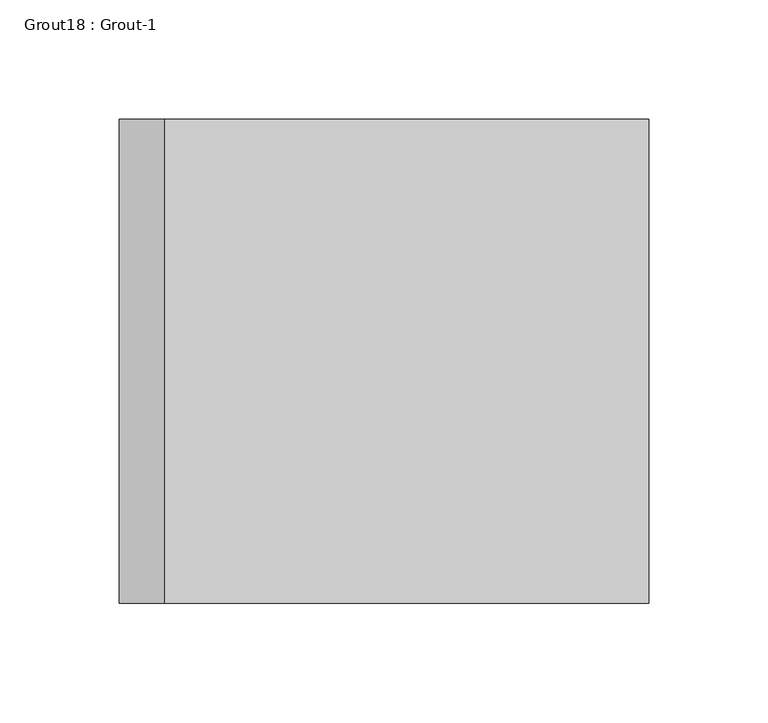
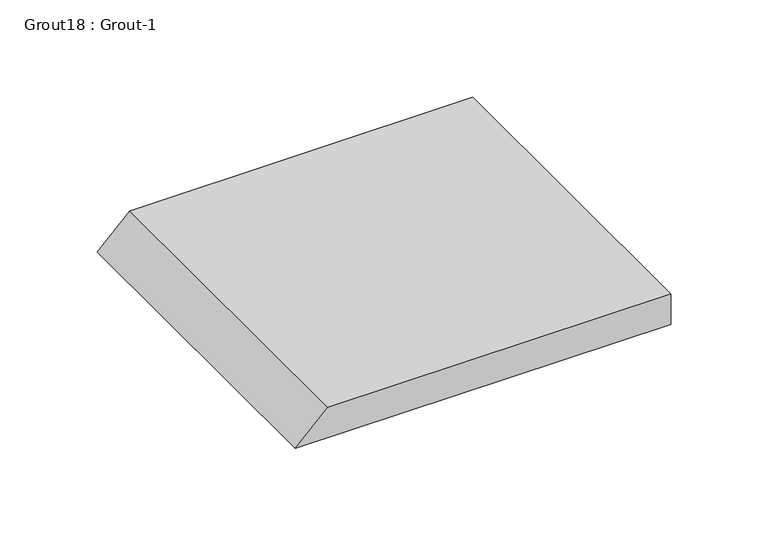
"""IFC4 building model written with IfcOpenShell, lengths in millimetres: proxy geometry, Grout18 : Grout-1."""

import ifcopenshell
import ifcopenshell.guid

model = None  # the IFC model being written
_history = None  # IfcOwnerHistory: only IFC2X3 demands one
_inside = {}  # id of a spatial element -> (the spatial element, [elements in it])
_under = {}  # id of a project, library or spatial element -> (it, [spatial elements below it])
_declared = {}  # id of a project -> (the project, [libraries it declares])
_typed = {}  # id of a type object -> (the type object, [elements of that type])
_made_of = {}  # id of a material, layer set ... -> (it, [elements and type objects made of it])


def new_model(schema):
    """Start an empty IFC model of exactly this schema.

    Asked for "IFC4X3", IfcOpenShell would pick the latest addendum, in which some entities
    have other attributes; the version numbers below select the first issue.
    IFC2X3 requires an IfcOwnerHistory on every rooted entity: one is made here for all.
    """
    global model, _history
    if schema == "IFC4X3":
        model = ifcopenshell.file(schema_version=(4, 3, 0, 0))
    else:
        model = ifcopenshell.file(schema=schema)
    _inside.clear()
    _under.clear()
    _declared.clear()
    _typed.clear()
    _made_of.clear()
    _history = None
    if model.schema == "IFC2X3":
        org = make("IfcOrganization", Name="unknown")
        user = make(
            "IfcPersonAndOrganization",
            ThePerson=make("IfcPerson", FamilyName="unknown"),
            TheOrganization=org,
        )
        app = make(
            "IfcApplication",
            ApplicationDeveloper=org,
            Version="unknown",
            ApplicationFullName="unknown",
            ApplicationIdentifier="unknown",
        )
        _history = make(
            "IfcOwnerHistory",
            OwningUser=user,
            OwningApplication=app,
            ChangeAction="ADDED",
            CreationDate=0,
        )
    return model


def make(cls, **values):
    """One entity of the class cls with the attributes given. An attribute that is None is left unset."""
    return model.create_entity(
        cls, **{name: value for name, value in values.items() if value is not None}
    )


def rooted(cls, **values):
    """An entity with a GlobalId (a new one), such as an element, a storey or a relation."""
    return make(cls, GlobalId=ifcopenshell.guid.new(), OwnerHistory=_history, **values)


def si_unit(unit_type, name, prefix=None):
    """IfcSIUnit, for example si_unit("LENGTHUNIT", "METRE", prefix="MILLI")."""
    return make("IfcSIUnit", UnitType=unit_type, Prefix=prefix, Name=name)


def assignment(units):
    """IfcUnitAssignment: the units of a project."""
    return None if units is None else make("IfcUnitAssignment", Units=units)


def point(xyz):
    """IfcCartesianPoint."""
    return None if xyz is None else make("IfcCartesianPoint", Coordinates=xyz)


def direction(xyz):
    """IfcDirection."""
    return None if xyz is None else make("IfcDirection", DirectionRatios=xyz)


def frame(location, z_axis=None, x_axis=None):
    """IfcAxis2Placement3D, a coordinate frame: its origin and axes. An axis left out is left unset."""
    return make(
        "IfcAxis2Placement3D",
        Location=point(location),
        Axis=direction(z_axis),
        RefDirection=direction(x_axis),
    )


def origin():
    """The frame at (0, 0, 0) with its axes left unset."""
    return frame((0.0, 0.0, 0.0))


def place(relative_to, where):
    """IfcLocalPlacement: puts the frame where relative to a parent placement (None: the world)."""
    return make(
        "IfcLocalPlacement", PlacementRelTo=relative_to, RelativePlacement=where
    )


def context(
    kind, dimensions, precision=None, world=None, true_north=None, identifier=None
):
    """IfcGeometricRepresentationContext, for example the 3D "Model" context."""
    return make(
        "IfcGeometricRepresentationContext",
        ContextIdentifier=identifier,
        ContextType=kind,
        CoordinateSpaceDimension=dimensions,
        Precision=precision,
        WorldCoordinateSystem=world,
        TrueNorth=true_north,
    )


def project(units=None, contexts=None):
    """IfcProject with its units and contexts."""
    return rooted(
        "IfcProject",
        Name="project",
        RepresentationContexts=contexts,
        UnitsInContext=assignment(units),
    )


def spatial(cls, under=None, at=None, **own):
    """A site, building, storey or space (cls), placed at a placement, below another one or the project."""
    s = rooted(cls, ObjectPlacement=at, **own)
    if under is not None:
        _under.setdefault(under.id(), (under, []))[1].append(s)
    return s


def polyline(points):
    """IfcPolyline through the points."""
    return make("IfcPolyline", Points=[point(p) for p in points])


def outline(outer, holes=None, kind="AREA"):
    """IfcArbitraryClosedProfileDef: a profile drawn as a closed curve; with holes, ...WithVoids."""
    if holes is None:
        return make("IfcArbitraryClosedProfileDef", ProfileType=kind, OuterCurve=outer)
    return make(
        "IfcArbitraryProfileDefWithVoids",
        ProfileType=kind,
        OuterCurve=outer,
        InnerCurves=holes,
    )


def extrude(swept, where, along, depth):
    """IfcExtrudedAreaSolid: the profile swept, set in the frame where, extruded along a direction by depth."""
    return make(
        "IfcExtrudedAreaSolid",
        SweptArea=swept,
        Position=where,
        ExtrudedDirection=direction(along),
        Depth=depth,
    )


def shape(context_of_items, identifier, shape_type, items):
    """IfcShapeRepresentation: the items that make up one representation, for example the "Body"."""
    return make(
        "IfcShapeRepresentation",
        ContextOfItems=context_of_items,
        RepresentationIdentifier=identifier,
        RepresentationType=shape_type,
        Items=items,
    )


def source(mapping_origin, context_of_items, identifier, shape_type, items):
    """IfcRepresentationMap: a shape defined once, which mapped items show again and again."""
    return make(
        "IfcRepresentationMap",
        MappingOrigin=mapping_origin,
        MappedRepresentation=shape(context_of_items, identifier, shape_type, items),
    )


def transform(
    local_origin,
    x_axis=None,
    y_axis=None,
    z_axis=None,
    scale=None,
    scale2=None,
    scale3=None,
    uniform=True,
):
    """IfcCartesianTransformationOperator3D, or its non-uniform kind. x_axis, y_axis, z_axis: its Axis1, 2, 3."""
    if uniform:
        return make(
            "IfcCartesianTransformationOperator3D",
            Axis1=direction(x_axis),
            Axis2=direction(y_axis),
            LocalOrigin=point(local_origin),
            Scale=scale,
            Axis3=direction(z_axis),
        )
    return make(
        "IfcCartesianTransformationOperator3DnonUniform",
        Axis1=direction(x_axis),
        Axis2=direction(y_axis),
        LocalOrigin=point(local_origin),
        Scale=scale,
        Axis3=direction(z_axis),
        Scale2=scale2,
        Scale3=scale3,
    )


def mapped(mapping_source, mapping_target):
    """IfcMappedItem: shows the shape of a source again, moved by a transform."""
    return make(
        "IfcMappedItem", MappingSource=mapping_source, MappingTarget=mapping_target
    )


def made_of(thing, what):
    """Note that an element or type object is made of a material, layer set ...; save() writes the relation."""
    if what is not None:
        _made_of.setdefault(what.id(), (what, []))[1].append(thing)
    return thing


def element(
    cls,
    number,
    at=None,
    inside=None,
    cuts=None,
    type_object=None,
    material=None,
    context=None,
    identifier="Body",
    shape_type=None,
    held_by="IfcProductDefinitionShape",
    body=None,
    shapes=None,
    **own,
):
    """One element of the class cls, such as IfcWall. Its Tag is "e" and its number.

    at: its placement. inside: the storey or other place that contains it. cuts: it is an
    opening in that element (IfcRelVoidsElement). A single representation is given by context,
    identifier, shape_type and body (its items); several are given by shapes. held_by: the class
    of the entity that holds the representations. save() writes the other relations.
    """
    e = rooted(cls, Tag="e%d" % number, ObjectPlacement=at, **own)
    if body is not None:
        shapes = [shape(context, identifier, shape_type, body)]
    if shapes is not None:
        e.Representation = make(held_by, Representations=shapes)
    if inside is not None:
        _inside.setdefault(inside.id(), (inside, []))[1].append(e)
    if cuts is not None:
        rooted(
            "IfcRelVoidsElement", RelatingBuildingElement=cuts, RelatedOpeningElement=e
        )
    if type_object is not None:
        _typed.setdefault(type_object.id(), (type_object, []))[1].append(e)
    return made_of(e, material)


def aggregate(whole, parts):
    """IfcRelAggregates: a whole, such as a stair, and the parts it consists of."""
    return rooted("IfcRelAggregates", RelatingObject=whole, RelatedObjects=parts)


def save(model, path):
    """Write the relations noted so far, then the file.

    IfcRelAggregates (storeys below a building ...), IfcRelContainedInSpatialStructure (elements
    in a storey), IfcRelDefinesByType, IfcRelAssociatesMaterial and IfcRelDeclares: one each for
    every whole, place, type object, material and project.
    """
    for whole, parts in _under.values():
        aggregate(whole, parts)
    for where, things in _inside.values():
        rooted(
            "IfcRelContainedInSpatialStructure",
            RelatedElements=things,
            RelatingStructure=where,
        )
    for kind, things in _typed.values():
        rooted("IfcRelDefinesByType", RelatedObjects=things, RelatingType=kind)
    for what, things in _made_of.values():
        rooted("IfcRelAssociatesMaterial", RelatedObjects=things, RelatingMaterial=what)
    for by, libraries in _declared.values():
        rooted("IfcRelDeclares", RelatingContext=by, RelatedDefinitions=libraries)
    model.write(path)


def grout18_grout_1_248e8b60(model_context):
    return source(origin(), model_context, "Body", "SweptSolid", [
        extrude(outline(polyline([(19.05, 590115.4434739), (0.0, 590096.3934739), (0.0, 590318.6434739), (19.05, 590318.6434739), (19.05, 590115.4434739)])), frame((0.0, -536468.3913841, 0.0), z_axis=(0.0, 1.0, 0.0), x_axis=(0.0, 0.0, 1.0)), (0.0, 0.0, 1.0), 203.2),
    ])


if __name__ == "__main__":
    model = new_model("IFC4")
    model_context = context("Model", 3, world=origin())
    ifc_project = project(units=[si_unit("LENGTHUNIT", "METRE", prefix="MILLI")], contexts=[model_context])
    site = spatial("IfcSite", under=ifc_project)
    building = spatial("IfcBuilding", under=site)
    placement = place(None, origin())
    grout18_grout_1_shape = grout18_grout_1_248e8b60(model_context)
    element("IfcBuildingElementProxy", 1, Name="Grout18 : Grout-1", ObjectType="Grout18 : Grout-1", at=placement, inside=building, context=model_context, shape_type="MappedRepresentation", body=[
        mapped(grout18_grout_1_shape, transform((0.0, 0.0, 0.0), x_axis=(1.0, 0.0, 0.0), y_axis=(0.0, 1.0, 0.0), z_axis=(0.0, 0.0, 1.0))),
    ])
    save(model, "model.ifc")

# Revit data of these elements
# Element 1 (IfcBuildingElementProxy, "Grout18 : Grout-1")
#   Materials on its faces: "3/4\" NON SHRINK GROUT"
# Materials
#   "3/4\" NON SHRINK GROUT": class "Generic", colour RGB 145 145 143, transparency 0, Cost = 0
